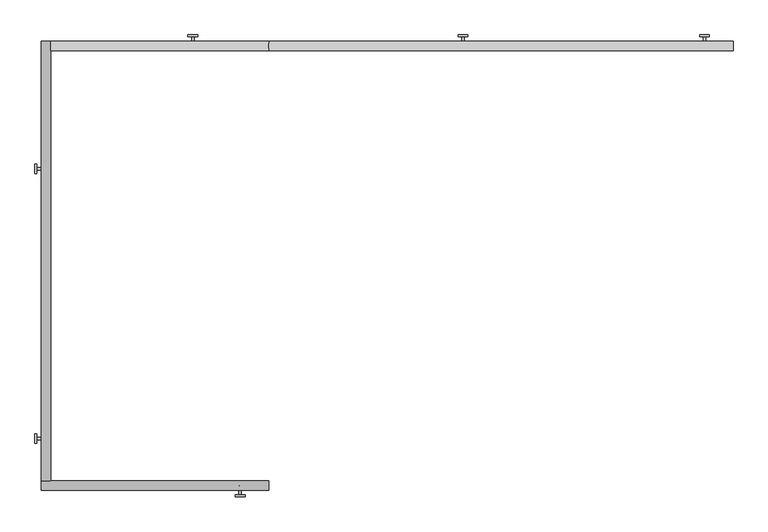
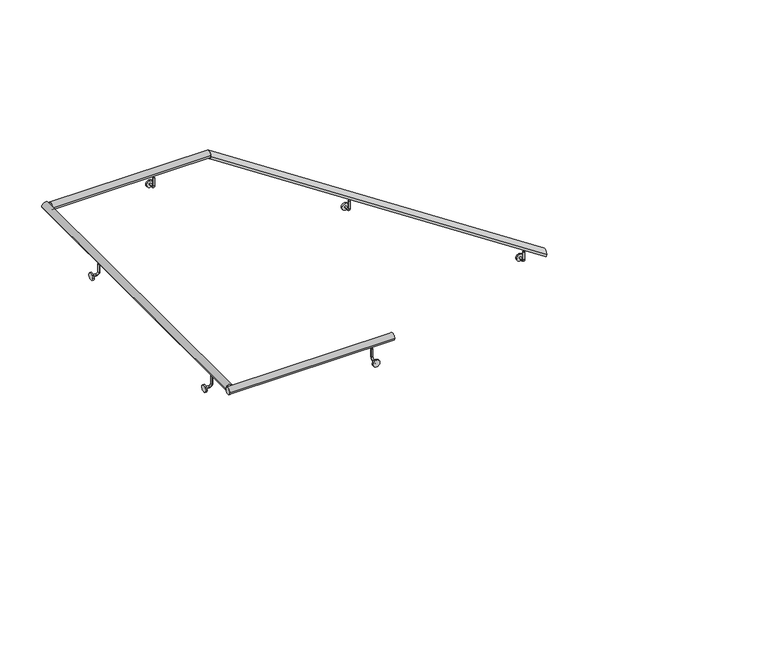
"""IFC4 building model written with IfcOpenShell, lengths in millimetres: railing geometry."""

from ifc_helpers import new_model, si_unit, point, frame, frame_2d, origin, place, context, project, spatial, circle_curve, ellipse_curve, trimmed, segment, composite_curve, outline, extrude, source, transform, mapped, element, save
from ifc_brep_helpers import plane_surface, cylinder_surface, revolved_surface, advanced_brep


def railing_2f2e9fd8(model_context):
    return source(origin(), model_context, "Body", "SolidModel", [
        advanced_brep(
        [(-47841.1127262, 17739.1574868, 1147.8451634), (-47841.1127262, 17789.1574868, 1147.8451634), (-50271.1127262, 17739.1574868, 2747.8451634), (-50271.1127262, 17789.1574868, 2747.8451634)],
        [
            (0, 1, ellipse_curve(frame((-47841.1127262, 17764.1574868, 1147.8451634), z_axis=(1.0, 0.0, 0.0), x_axis=(0.0, 0.0, -1.0)), 29.9326144, 25.0)),
            (1, 0, ellipse_curve(frame((-47841.1127262, 17764.1574868, 1147.8451634), z_axis=(1.0, 0.0, 0.0), x_axis=(0.0, 0.0, -1.0)), 29.9326144, 25.0)),
            (2, 3, ellipse_curve(frame((-50271.1127262, 17764.1574868, 2747.8451634), z_axis=(-1.0, 0.0, 0.0), x_axis=(0.0, 0.0, -1.0)), 29.9326144, 25.0)),
            (3, 2, ellipse_curve(frame((-50271.1127262, 17764.1574868, 2747.8451634), z_axis=(-1.0, 0.0, 0.0), x_axis=(0.0, 0.0, -1.0)), 29.9326144, 25.0)),
            (0, 2),
            (3, 1),
        ],
        [
            plane_surface(frame((-47841.1127262, 17764.1574868, 1177.7777778), z_axis=(1.0, 0.0, 0.0), x_axis=(0.0, -1.0, 0.0))),
            plane_surface(frame((-50271.1127262, 17764.1574868, 2777.7777778), z_axis=(-1.0, 0.0, 0.0), x_axis=(0.0, -1.0, 0.0))),
            cylinder_surface(frame((-47854.8610286, 17764.1574868, 1156.8975435), z_axis=(0.8352093694289686, 0.0, -0.5499320950972626), x_axis=(0.0, 1.0, 0.0)), 25.0),
        ],
        [
            (0, [[1, 2]]),
            (1, [[3, 4]]),
            (2, [[-1, 5, -4, 6]]),
            (2, [[-2, -6, -3, -5]]),
        ],
    ),
        advanced_brep(
        [(-50271.1127262, 17739.1574868, 2752.7777778), (-50271.1127262, 17789.1574868, 2752.7777778), (-51413.5127262, 17739.1574868, 2752.7777778), (-51413.5127262, 17789.1574868, 2752.7777778)],
        [
            (0, 1, circle_curve(frame((-50271.1127262, 17764.1574868, 2752.7777778), z_axis=(1.0, 0.0, 0.0), x_axis=(0.0, 1.0, 0.0)), 25.0)),
            (1, 0, circle_curve(frame((-50271.1127262, 17764.1574868, 2752.7777778), z_axis=(1.0, 0.0, 0.0), x_axis=(0.0, 1.0, 0.0)), 25.0)),
            (2, 3, circle_curve(frame((-51413.5127262, 17764.1574868, 2752.7777778), z_axis=(-1.0, 0.0, 0.0), x_axis=(0.0, 1.0, 0.0)), 25.0)),
            (3, 2, circle_curve(frame((-51413.5127262, 17764.1574868, 2752.7777778), z_axis=(-1.0, 0.0, 0.0), x_axis=(0.0, 1.0, 0.0)), 25.0)),
            (0, 2),
            (3, 1),
        ],
        [
            plane_surface(frame((-50271.1127262, 17764.1574868, 2777.7777778), z_axis=(1.0, 0.0, 0.0), x_axis=(0.0, -1.0, 0.0))),
            plane_surface(frame((-51413.5127262, 17764.1574868, 2777.7777778), z_axis=(-1.0, 0.0, 0.0), x_axis=(0.0, -1.0, 0.0))),
            cylinder_surface(frame((-50271.1127262, 17764.1574868, 2752.7777778), z_axis=(1.0, 0.0, 0.0), x_axis=(0.0, 1.0, 0.0)), 25.0),
        ],
        [
            (0, [[1, 2]]),
            (1, [[3, 4]]),
            (2, [[-1, 5, -4, 6]]),
            (2, [[-2, -6, -3, -5]]),
        ],
    ),
        advanced_brep(
        [(-51413.5127262, 17789.1574868, 2752.7777778), (-51463.5127262, 17789.1574868, 2752.7777778), (-51413.5127262, 15484.3587092, 2752.7777778), (-51463.5127262, 15484.3587092, 2752.7777778)],
        [
            (0, 1, circle_curve(frame((-51438.5127262, 17789.1574868, 2752.7777778), z_axis=(0.0, 1.0, 0.0), x_axis=(-1.0, 0.0, 0.0)), 25.0)),
            (1, 0, circle_curve(frame((-51438.5127262, 17789.1574868, 2752.7777778), z_axis=(0.0, 1.0, 0.0), x_axis=(-1.0, 0.0, 0.0)), 25.0)),
            (2, 3, circle_curve(frame((-51438.5127262, 15484.3587092, 2752.7777778), z_axis=(0.0, -1.0, 0.0), x_axis=(-1.0, 0.0, 0.0)), 25.0)),
            (3, 2, circle_curve(frame((-51438.5127262, 15484.3587092, 2752.7777778), z_axis=(0.0, -1.0, 0.0), x_axis=(-1.0, 0.0, 0.0)), 25.0)),
            (0, 2),
            (3, 1),
        ],
        [
            plane_surface(frame((-51438.5127262, 17789.1574868, 2777.7777778), z_axis=(0.0, 1.0, 0.0), x_axis=(0.0, 0.0, -1.0))),
            plane_surface(frame((-51438.5127262, 15484.3587092, 2777.7777778), z_axis=(0.0, -1.0, 0.0), x_axis=(0.0, 0.0, -1.0))),
            cylinder_surface(frame((-51438.5127262, 17789.1574868, 2752.7777778), z_axis=(0.0, 1.0, 0.0), x_axis=(-1.0, 0.0, 0.0)), 25.0),
        ],
        [
            (0, [[1, 2]]),
            (1, [[3, 4]]),
            (2, [[-1, 5, -4, 6]]),
            (2, [[-2, -6, -3, -5]]),
        ],
    ),
        advanced_brep(
        [(-51463.5127262, 15484.3587092, 2752.7777778), (-51463.5127262, 15434.3587092, 2752.7777778), (-50271.1127262, 15484.3587092, 2752.7777778), (-50271.1127262, 15434.3587092, 2752.7777778)],
        [
            (0, 1, circle_curve(frame((-51463.5127262, 15459.3587092, 2752.7777778), z_axis=(-1.0, 0.0, 0.0), x_axis=(0.0, -1.0, 0.0)), 25.0)),
            (1, 0, circle_curve(frame((-51463.5127262, 15459.3587092, 2752.7777778), z_axis=(-1.0, 0.0, 0.0), x_axis=(0.0, -1.0, 0.0)), 25.0)),
            (2, 3, circle_curve(frame((-50271.1127262, 15459.3587092, 2752.7777778), z_axis=(1.0, 0.0, 0.0), x_axis=(0.0, -1.0, 0.0)), 25.0)),
            (3, 2, circle_curve(frame((-50271.1127262, 15459.3587092, 2752.7777778), z_axis=(1.0, 0.0, 0.0), x_axis=(0.0, -1.0, 0.0)), 25.0)),
            (0, 2),
            (3, 1),
        ],
        [
            plane_surface(frame((-51463.5127262, 15459.3587092, 2777.7777778), z_axis=(-1.0, 0.0, 0.0), x_axis=(0.0, 1.0, 0.0))),
            plane_surface(frame((-50271.1127262, 15459.3587092, 2777.7777778), z_axis=(1.0, 0.0, 0.0), x_axis=(0.0, 1.0, 0.0))),
            cylinder_surface(frame((-51463.5127262, 15459.3587092, 2752.7777778), z_axis=(-1.0, 0.0, 0.0), x_axis=(0.0, -1.0, 0.0)), 25.0),
        ],
        [
            (0, [[1, 2]]),
            (1, [[3, 4]]),
            (2, [[-1, 5, -4, 6]]),
            (2, [[-2, -6, -3, -5]]),
        ],
    ),
        advanced_brep(
        [(-51438.5127262, 15712.2284647, 2708.7277778), (-51438.5127262, 15699.5284647, 2708.7277778), (-51438.5127262, 15712.2284647, 2651.5777778), (-51438.5127262, 15699.5284647, 2651.5777778), (-51457.5627262, 15699.5284647, 2632.5277778), (-51457.5627262, 15712.2284647, 2632.5277778), (-51486.1377262, 15712.2284647, 2632.5277778), (-51486.1377262, 15699.5284647, 2632.5277778)],
        [
            (0, 1, circle_curve(frame((-51438.5127262, 15705.8784647, 2708.7277778), z_axis=(0.0, 0.0, 1.0), x_axis=(0.0, -1.0, 0.0)), 6.35)),
            (1, 0, circle_curve(frame((-51438.5127262, 15705.8784647, 2708.7277778), z_axis=(0.0, 0.0, 1.0), x_axis=(0.0, -1.0, 0.0)), 6.35)),
            (0, 2),
            (2, 3, circle_curve(frame((-51438.5127262, 15705.8784647, 2651.5777778), z_axis=(0.0, 0.0, 1.0), x_axis=(0.0, -1.0, 0.0)), 6.35)),
            (3, 1),
            (3, 2, circle_curve(frame((-51438.5127262, 15705.8784647, 2651.5777778), z_axis=(0.0, 0.0, 1.0), x_axis=(0.0, -1.0, 0.0)), 6.35)),
            (4, 3, circle_curve(frame((-51457.5627262, 15699.5284647, 2651.5777778), z_axis=(0.0, -1.0, 0.0), x_axis=(1.0, 0.0, 0.0)), 19.05)),
            (2, 5, circle_curve(frame((-51457.5627262, 15712.2284647, 2651.5777778), z_axis=(0.0, 1.0, 0.0), x_axis=(1.0, 0.0, 0.0)), 19.05)),
            (5, 4, circle_curve(frame((-51457.5627262, 15705.8784647, 2632.5277778), z_axis=(1.0, 0.0, 0.0), x_axis=(0.0, -1.0, 0.0)), 6.35)),
            (4, 5, circle_curve(frame((-51457.5627262, 15705.8784647, 2632.5277778), z_axis=(1.0, 0.0, 0.0), x_axis=(0.0, -1.0, 0.0)), 6.35)),
            (6, 7, circle_curve(frame((-51486.1377262, 15705.8784647, 2632.5277778), z_axis=(-1.0, 0.0, 0.0), x_axis=(0.0, -1.0, 0.0)), 6.35)),
            (7, 6, circle_curve(frame((-51486.1377262, 15705.8784647, 2632.5277778), z_axis=(-1.0, 0.0, 0.0), x_axis=(0.0, -1.0, 0.0)), 6.35)),
            (5, 6),
            (7, 4),
        ],
        [
            plane_surface(frame((-51438.5127262, 15699.5284647, 2708.7277778), z_axis=(0.0, 0.0, 1.0), x_axis=(-1.0, 0.0, 0.0))),
            cylinder_surface(frame((-51438.5127262, 15705.8784647, 2708.7277778), z_axis=(0.0, 0.0, 1.0), x_axis=(0.0, -1.0, 0.0)), 6.35),
            revolved_surface(trimmed(ellipse_curve(frame((-51438.5127262, 15705.8784647, 2651.5777778), z_axis=(0.0, 0.0, 1.0), x_axis=(0.0, -1.0, 0.0)), 6.35, 6.35), [point((-51438.5127262, 15712.2284647, 2651.5777778))], [point((-51438.5127262, 15699.5284647, 2651.5777778))], True, "CARTESIAN"), (-51457.5627262, 15705.8784647, 2651.5777778), (0.0, 1.0, 0.0)),
            revolved_surface(trimmed(ellipse_curve(frame((-51438.5127262, 15705.8784647, 2651.5777778), z_axis=(0.0, 0.0, 1.0), x_axis=(0.0, -1.0, 0.0)), 6.35, 6.35), [point((-51438.5127262, 15699.5284647, 2651.5777778))], [point((-51438.5127262, 15712.2284647, 2651.5777778))], True, "CARTESIAN"), (-51457.5627262, 15705.8784647, 2651.5777778), (0.0, 1.0, 0.0)),
            plane_surface(frame((-51486.1377262, 15705.8784647, 2626.1777778), z_axis=(-1.0, 0.0, 0.0), x_axis=(0.0, -1.0, 0.0))),
            cylinder_surface(frame((-51457.5627262, 15705.8784647, 2632.5277778), z_axis=(1.0, 0.0, 0.0), x_axis=(0.0, -1.0, 0.0)), 6.35),
        ],
        [
            (0, [[1, 2]]),
            (1, [[-1, 3, 4, 5]]),
            (1, [[-2, -5, 6, -3]]),
            (2, [[7, -4, 8, 9]]),
            (3, [[-8, -6, -7, 10]]),
            (4, [[11, 12]]),
            (5, [[-9, 13, -12, 14]]),
            (5, [[-10, -14, -11, -13]]),
        ],
    ),
        extrude(outline(composite_curve([segment(trimmed(circle_curve(frame_2d((15705.8784647, 2632.5277778)), 25.4), [point((15680.4784647, 2632.5277778))], [point((15731.2784647, 2632.5277778))], False, "CARTESIAN"), True, "CONTINUOUS"), segment(trimmed(circle_curve(frame_2d((15705.8784647, 2632.5277778)), 25.4), [point((15731.2784647, 2632.5277778))], [point((15680.4784647, 2632.5277778))], False, "CARTESIAN"), True, "CONTINUOUS")], self_intersect=False)), frame((-51495.6627262, 0.0, 0.0), z_axis=(1.0, 0.0, 0.0), x_axis=(0.0, 1.0, 0.0)), (0.0, 0.0, 1.0), 9.525),
        advanced_brep(
        [(-51438.5127262, 17126.1482202, 2708.7277778), (-51438.5127262, 17113.4482202, 2708.7277778), (-51438.5127262, 17126.1482202, 2651.5777778), (-51438.5127262, 17113.4482202, 2651.5777778), (-51457.5627262, 17113.4482202, 2632.5277778), (-51457.5627262, 17126.1482202, 2632.5277778), (-51486.1377262, 17126.1482202, 2632.5277778), (-51486.1377262, 17113.4482202, 2632.5277778)],
        [
            (0, 1, circle_curve(frame((-51438.5127262, 17119.7982202, 2708.7277778), z_axis=(0.0, 0.0, 1.0), x_axis=(0.0, -1.0, 0.0)), 6.35)),
            (1, 0, circle_curve(frame((-51438.5127262, 17119.7982202, 2708.7277778), z_axis=(0.0, 0.0, 1.0), x_axis=(0.0, -1.0, 0.0)), 6.35)),
            (0, 2),
            (2, 3, circle_curve(frame((-51438.5127262, 17119.7982202, 2651.5777778), z_axis=(0.0, 0.0, 1.0), x_axis=(0.0, -1.0, 0.0)), 6.35)),
            (3, 1),
            (3, 2, circle_curve(frame((-51438.5127262, 17119.7982202, 2651.5777778), z_axis=(0.0, 0.0, 1.0), x_axis=(0.0, -1.0, 0.0)), 6.35)),
            (4, 3, circle_curve(frame((-51457.5627262, 17113.4482202, 2651.5777778), z_axis=(0.0, -1.0, 0.0), x_axis=(1.0, 0.0, 0.0)), 19.05)),
            (2, 5, circle_curve(frame((-51457.5627262, 17126.1482202, 2651.5777778), z_axis=(0.0, 1.0, 0.0), x_axis=(1.0, 0.0, 0.0)), 19.05)),
            (5, 4, circle_curve(frame((-51457.5627262, 17119.7982202, 2632.5277778), z_axis=(1.0, 0.0, 0.0), x_axis=(0.0, -1.0, 0.0)), 6.35)),
            (4, 5, circle_curve(frame((-51457.5627262, 17119.7982202, 2632.5277778), z_axis=(1.0, 0.0, 0.0), x_axis=(0.0, -1.0, 0.0)), 6.35)),
            (6, 7, circle_curve(frame((-51486.1377262, 17119.7982202, 2632.5277778), z_axis=(-1.0, 0.0, 0.0), x_axis=(0.0, -1.0, 0.0)), 6.35)),
            (7, 6, circle_curve(frame((-51486.1377262, 17119.7982202, 2632.5277778), z_axis=(-1.0, 0.0, 0.0), x_axis=(0.0, -1.0, 0.0)), 6.35)),
            (5, 6),
            (7, 4),
        ],
        [
            plane_surface(frame((-51438.5127262, 17113.4482202, 2708.7277778), z_axis=(0.0, 0.0, 1.0), x_axis=(-1.0, 0.0, 0.0))),
            cylinder_surface(frame((-51438.5127262, 17119.7982202, 2708.7277778), z_axis=(0.0, 0.0, 1.0), x_axis=(0.0, -1.0, 0.0)), 6.35),
            revolved_surface(trimmed(ellipse_curve(frame((-51438.5127262, 17119.7982202, 2651.5777778), z_axis=(0.0, 0.0, 1.0), x_axis=(0.0, -1.0, 0.0)), 6.35, 6.35), [point((-51438.5127262, 17126.1482202, 2651.5777778))], [point((-51438.5127262, 17113.4482202, 2651.5777778))], True, "CARTESIAN"), (-51457.5627262, 17119.7982202, 2651.5777778), (0.0, 1.0, 0.0)),
            revolved_surface(trimmed(ellipse_curve(frame((-51438.5127262, 17119.7982202, 2651.5777778), z_axis=(0.0, 0.0, 1.0), x_axis=(0.0, -1.0, 0.0)), 6.35, 6.35), [point((-51438.5127262, 17113.4482202, 2651.5777778))], [point((-51438.5127262, 17126.1482202, 2651.5777778))], True, "CARTESIAN"), (-51457.5627262, 17119.7982202, 2651.5777778), (0.0, 1.0, 0.0)),
            plane_surface(frame((-51486.1377262, 17119.7982202, 2626.1777778), z_axis=(-1.0, 0.0, 0.0), x_axis=(0.0, -1.0, 0.0))),
            cylinder_surface(frame((-51457.5627262, 17119.7982202, 2632.5277778), z_axis=(1.0, 0.0, 0.0), x_axis=(0.0, -1.0, 0.0)), 6.35),
        ],
        [
            (0, [[1, 2]]),
            (1, [[-1, 3, 4, 5]]),
            (1, [[-2, -5, 6, -3]]),
            (2, [[7, -4, 8, 9]]),
            (3, [[-8, -6, -7, 10]]),
            (4, [[11, 12]]),
            (5, [[-9, 13, -12, 14]]),
            (5, [[-10, -14, -11, -13]]),
        ],
    ),
        extrude(outline(composite_curve([segment(trimmed(circle_curve(frame_2d((17119.7982202, 2632.5277778)), 25.4), [point((17094.3982202, 2632.5277778))], [point((17145.1982202, 2632.5277778))], False, "CARTESIAN"), True, "CONTINUOUS"), segment(trimmed(circle_curve(frame_2d((17119.7982202, 2632.5277778)), 25.4), [point((17145.1982202, 2632.5277778))], [point((17094.3982202, 2632.5277778))], False, "CARTESIAN"), True, "CONTINUOUS")], self_intersect=False)), frame((-51495.6627262, 0.0, 0.0), z_axis=(1.0, 0.0, 0.0), x_axis=(0.0, 1.0, 0.0)), (0.0, 0.0, 1.0), 9.525),
        advanced_brep(
        [(-50662.6022373, 17764.1574868, 2708.7277778), (-50675.3022373, 17764.1574868, 2708.7277778), (-50662.6022373, 17764.1574868, 2651.5777778), (-50675.3022373, 17764.1574868, 2651.5777778), (-50675.3022373, 17783.2074868, 2632.5277778), (-50662.6022373, 17783.2074868, 2632.5277778), (-50662.6022373, 17811.7824868, 2632.5277778), (-50675.3022373, 17811.7824868, 2632.5277778)],
        [
            (0, 1, circle_curve(frame((-50668.9522373, 17764.1574868, 2708.7277778), z_axis=(0.0, 0.0, 1.0), x_axis=(-1.0, 0.0, 0.0)), 6.35)),
            (1, 0, circle_curve(frame((-50668.9522373, 17764.1574868, 2708.7277778), z_axis=(0.0, 0.0, 1.0), x_axis=(-1.0, 0.0, 0.0)), 6.35)),
            (0, 2),
            (2, 3, circle_curve(frame((-50668.9522373, 17764.1574868, 2651.5777778), z_axis=(0.0, 0.0, 1.0), x_axis=(-1.0, 0.0, 0.0)), 6.35)),
            (3, 1),
            (3, 2, circle_curve(frame((-50668.9522373, 17764.1574868, 2651.5777778), z_axis=(0.0, 0.0, 1.0), x_axis=(-1.0, 0.0, 0.0)), 6.35)),
            (4, 3, circle_curve(frame((-50675.3022373, 17783.2074868, 2651.5777778), z_axis=(-1.0, 0.0, 0.0), x_axis=(0.0, -1.0, 0.0)), 19.05)),
            (2, 5, circle_curve(frame((-50662.6022373, 17783.2074868, 2651.5777778), z_axis=(1.0, 0.0, 0.0), x_axis=(0.0, -1.0, 0.0)), 19.05)),
            (5, 4, circle_curve(frame((-50668.9522373, 17783.2074868, 2632.5277778), z_axis=(0.0, -1.0, 0.0), x_axis=(-1.0, 0.0, 0.0)), 6.35)),
            (4, 5, circle_curve(frame((-50668.9522373, 17783.2074868, 2632.5277778), z_axis=(0.0, -1.0, 0.0), x_axis=(-1.0, 0.0, 0.0)), 6.35)),
            (6, 7, circle_curve(frame((-50668.9522373, 17811.7824868, 2632.5277778), z_axis=(0.0, 1.0, 0.0), x_axis=(-1.0, 0.0, 0.0)), 6.35)),
            (7, 6, circle_curve(frame((-50668.9522373, 17811.7824868, 2632.5277778), z_axis=(0.0, 1.0, 0.0), x_axis=(-1.0, 0.0, 0.0)), 6.35)),
            (5, 6),
            (7, 4),
        ],
        [
            plane_surface(frame((-50675.3022373, 17764.1574868, 2708.7277778), z_axis=(0.0, 0.0, 1.0), x_axis=(0.0, 1.0, 0.0))),
            cylinder_surface(frame((-50668.9522373, 17764.1574868, 2708.7277778), z_axis=(0.0, 0.0, 1.0), x_axis=(-1.0, 0.0, 0.0)), 6.35),
            revolved_surface(trimmed(ellipse_curve(frame((-50668.9522373, 17764.1574868, 2651.5777778), z_axis=(0.0, 0.0, 1.0), x_axis=(-1.0, 0.0, 0.0)), 6.35, 6.35), [point((-50662.6022373, 17764.1574868, 2651.5777778))], [point((-50675.3022373, 17764.1574868, 2651.5777778))], True, "CARTESIAN"), (-50668.9522373, 17783.2074868, 2651.5777778), (1.0, 0.0, 0.0)),
            revolved_surface(trimmed(ellipse_curve(frame((-50668.9522373, 17764.1574868, 2651.5777778), z_axis=(0.0, 0.0, 1.0), x_axis=(-1.0, 0.0, 0.0)), 6.35, 6.35), [point((-50675.3022373, 17764.1574868, 2651.5777778))], [point((-50662.6022373, 17764.1574868, 2651.5777778))], True, "CARTESIAN"), (-50668.9522373, 17783.2074868, 2651.5777778), (1.0, 0.0, 0.0)),
            plane_surface(frame((-50668.9522373, 17811.7824868, 2626.1777778), z_axis=(0.0, 1.0, 0.0), x_axis=(-1.0, 0.0, 0.0))),
            cylinder_surface(frame((-50668.9522373, 17783.2074868, 2632.5277778), z_axis=(0.0, -1.0, 0.0), x_axis=(-1.0, 0.0, 0.0)), 6.35),
        ],
        [
            (0, [[1, 2]]),
            (1, [[-1, 3, 4, 5]]),
            (1, [[-2, -5, 6, -3]]),
            (2, [[7, -4, 8, 9]]),
            (3, [[-8, -6, -7, 10]]),
            (4, [[11, 12]]),
            (5, [[-9, 13, -12, 14]]),
            (5, [[-10, -14, -11, -13]]),
        ],
    ),
        extrude(outline(composite_curve([segment(trimmed(circle_curve(frame_2d((2632.5277778, -50668.9522373)), 25.4), [point((2632.5277778, -50694.3522373))], [point((2632.5277778, -50643.5522373))], False, "CARTESIAN"), True, "CONTINUOUS"), segment(trimmed(circle_curve(frame_2d((2632.5277778, -50668.9522373)), 25.4), [point((2632.5277778, -50643.5522373))], [point((2632.5277778, -50694.3522373))], False, "CARTESIAN"), True, "CONTINUOUS")], self_intersect=False)), frame((0.0, 17811.7824868, 0.0), z_axis=(0.0, 1.0, 0.0), x_axis=(0.0, 0.0, 1.0)), (0.0, 0.0, 1.0), 9.525),
        advanced_brep(
        [(-49248.6824817, 17764.1574868, 2039.7037485), (-49261.3824817, 17764.1574868, 2039.7037485), (-49248.6824817, 17764.1574868, 1982.5537485), (-49261.3824817, 17764.1574868, 1982.5537485), (-49261.3824817, 17783.2074868, 1963.5037485), (-49248.6824817, 17783.2074868, 1963.5037485), (-49248.6824817, 17811.7824868, 1963.5037485), (-49261.3824817, 17811.7824868, 1963.5037485)],
        [
            (0, 1, circle_curve(frame((-49255.0324817, 17764.1574868, 2039.7037485), z_axis=(0.0, 0.0, 1.0), x_axis=(-1.0, 0.0, 0.0)), 6.35)),
            (1, 0, circle_curve(frame((-49255.0324817, 17764.1574868, 2039.7037485), z_axis=(0.0, 0.0, 1.0), x_axis=(-1.0, 0.0, 0.0)), 6.35)),
            (0, 2),
            (2, 3, circle_curve(frame((-49255.0324817, 17764.1574868, 1982.5537485), z_axis=(0.0, 0.0, 1.0), x_axis=(-1.0, 0.0, 0.0)), 6.35)),
            (3, 1),
            (3, 2, circle_curve(frame((-49255.0324817, 17764.1574868, 1982.5537485), z_axis=(0.0, 0.0, 1.0), x_axis=(-1.0, 0.0, 0.0)), 6.35)),
            (4, 3, circle_curve(frame((-49261.3824817, 17783.2074868, 1982.5537485), z_axis=(-1.0, 0.0, 0.0), x_axis=(0.0, -1.0, 0.0)), 19.05)),
            (2, 5, circle_curve(frame((-49248.6824817, 17783.2074868, 1982.5537485), z_axis=(1.0, 0.0, 0.0), x_axis=(0.0, -1.0, 0.0)), 19.05)),
            (5, 4, circle_curve(frame((-49255.0324817, 17783.2074868, 1963.5037485), z_axis=(0.0, -1.0, 0.0), x_axis=(-1.0, 0.0, 0.0)), 6.35)),
            (4, 5, circle_curve(frame((-49255.0324817, 17783.2074868, 1963.5037485), z_axis=(0.0, -1.0, 0.0), x_axis=(-1.0, 0.0, 0.0)), 6.35)),
            (6, 7, circle_curve(frame((-49255.0324817, 17811.7824868, 1963.5037485), z_axis=(0.0, 1.0, 0.0), x_axis=(-1.0, 0.0, 0.0)), 6.35)),
            (7, 6, circle_curve(frame((-49255.0324817, 17811.7824868, 1963.5037485), z_axis=(0.0, 1.0, 0.0), x_axis=(-1.0, 0.0, 0.0)), 6.35)),
            (5, 6),
            (7, 4),
        ],
        [
            plane_surface(frame((-49261.3824817, 17764.1574868, 2039.7037485), z_axis=(0.0, 0.0, 1.0), x_axis=(0.0, 1.0, 0.0))),
            cylinder_surface(frame((-49255.0324817, 17764.1574868, 2039.7037485), z_axis=(0.0, 0.0, 1.0), x_axis=(-1.0, 0.0, 0.0)), 6.35),
            revolved_surface(trimmed(ellipse_curve(frame((-49255.0324817, 17764.1574868, 1982.5537485), z_axis=(0.0, 0.0, 1.0), x_axis=(-1.0, 0.0, 0.0)), 6.35, 6.35), [point((-49248.6824817, 17764.1574868, 1982.5537485))], [point((-49261.3824817, 17764.1574868, 1982.5537485))], True, "CARTESIAN"), (-49255.0324817, 17783.2074868, 1982.5537485), (1.0, 0.0, 0.0)),
            revolved_surface(trimmed(ellipse_curve(frame((-49255.0324817, 17764.1574868, 1982.5537485), z_axis=(0.0, 0.0, 1.0), x_axis=(-1.0, 0.0, 0.0)), 6.35, 6.35), [point((-49261.3824817, 17764.1574868, 1982.5537485))], [point((-49248.6824817, 17764.1574868, 1982.5537485))], True, "CARTESIAN"), (-49255.0324817, 17783.2074868, 1982.5537485), (1.0, 0.0, 0.0)),
            plane_surface(frame((-49255.0324817, 17811.7824868, 1957.1537485), z_axis=(0.0, 1.0, 0.0), x_axis=(-1.0, 0.0, 0.0))),
            cylinder_surface(frame((-49255.0324817, 17783.2074868, 1963.5037485), z_axis=(0.0, -1.0, 0.0), x_axis=(-1.0, 0.0, 0.0)), 6.35),
        ],
        [
            (0, [[1, 2]]),
            (1, [[-1, 3, 4, 5]]),
            (1, [[-2, -5, 6, -3]]),
            (2, [[7, -4, 8, 9]]),
            (3, [[-8, -6, -7, 10]]),
            (4, [[11, 12]]),
            (5, [[-9, 13, -12, 14]]),
            (5, [[-10, -14, -11, -13]]),
        ],
    ),
        extrude(outline(composite_curve([segment(trimmed(circle_curve(frame_2d((1963.5037485, -49255.0324817)), 25.4), [point((1963.5037485, -49280.4324817))], [point((1963.5037485, -49229.6324817))], False, "CARTESIAN"), True, "CONTINUOUS"), segment(trimmed(circle_curve(frame_2d((1963.5037485, -49255.0324817)), 25.4), [point((1963.5037485, -49229.6324817))], [point((1963.5037485, -49280.4324817))], False, "CARTESIAN"), True, "CONTINUOUS")], self_intersect=False)), frame((0.0, 17811.7824868, 0.0), z_axis=(0.0, 1.0, 0.0), x_axis=(0.0, 0.0, 1.0)), (0.0, 0.0, 1.0), 9.525),
        advanced_brep(
        [(-50427.4627262, 15459.3587092, 2708.7277778), (-50414.7627262, 15459.3587092, 2708.7277778), (-50427.4627262, 15459.3587092, 2651.5777778), (-50414.7627262, 15459.3587092, 2651.5777778), (-50414.7627262, 15440.3087092, 2632.5277778), (-50427.4627262, 15440.3087092, 2632.5277778), (-50427.4627262, 15411.7337092, 2632.5277778), (-50414.7627262, 15411.7337092, 2632.5277778)],
        [
            (0, 1, circle_curve(frame((-50421.1127262, 15459.3587092, 2708.7277778), z_axis=(0.0, 0.0, 1.0), x_axis=(1.0, 0.0, 0.0)), 6.35)),
            (1, 0, circle_curve(frame((-50421.1127262, 15459.3587092, 2708.7277778), z_axis=(0.0, 0.0, 1.0), x_axis=(1.0, 0.0, 0.0)), 6.35)),
            (0, 2),
            (2, 3, circle_curve(frame((-50421.1127262, 15459.3587092, 2651.5777778), z_axis=(0.0, 0.0, 1.0), x_axis=(1.0, 0.0, 0.0)), 6.35)),
            (3, 1),
            (3, 2, circle_curve(frame((-50421.1127262, 15459.3587092, 2651.5777778), z_axis=(0.0, 0.0, 1.0), x_axis=(1.0, 0.0, 0.0)), 6.35)),
            (4, 3, circle_curve(frame((-50414.7627262, 15440.3087092, 2651.5777778), z_axis=(1.0, 0.0, 0.0), x_axis=(0.0, 1.0, 0.0)), 19.05)),
            (2, 5, circle_curve(frame((-50427.4627262, 15440.3087092, 2651.5777778), z_axis=(-1.0, 0.0, 0.0), x_axis=(0.0, 1.0, 0.0)), 19.05)),
            (5, 4, circle_curve(frame((-50421.1127262, 15440.3087092, 2632.5277778), z_axis=(0.0, 1.0, 0.0), x_axis=(1.0, 0.0, 0.0)), 6.35)),
            (4, 5, circle_curve(frame((-50421.1127262, 15440.3087092, 2632.5277778), z_axis=(0.0, 1.0, 0.0), x_axis=(1.0, 0.0, 0.0)), 6.35)),
            (6, 7, circle_curve(frame((-50421.1127262, 15411.7337092, 2632.5277778), z_axis=(0.0, -1.0, 0.0), x_axis=(1.0, 0.0, 0.0)), 6.35)),
            (7, 6, circle_curve(frame((-50421.1127262, 15411.7337092, 2632.5277778), z_axis=(0.0, -1.0, 0.0), x_axis=(1.0, 0.0, 0.0)), 6.35)),
            (5, 6),
            (7, 4),
        ],
        [
            plane_surface(frame((-50414.7627262, 15459.3587092, 2708.7277778), z_axis=(0.0, 0.0, 1.0), x_axis=(0.0, -1.0, 0.0))),
            cylinder_surface(frame((-50421.1127262, 15459.3587092, 2708.7277778), z_axis=(0.0, 0.0, 1.0), x_axis=(1.0, 0.0, 0.0)), 6.35),
            revolved_surface(trimmed(ellipse_curve(frame((-50421.1127262, 15459.3587092, 2651.5777778), z_axis=(0.0, 0.0, 1.0), x_axis=(1.0, 0.0, 0.0)), 6.35, 6.35), [point((-50427.4627262, 15459.3587092, 2651.5777778))], [point((-50414.7627262, 15459.3587092, 2651.5777778))], True, "CARTESIAN"), (-50421.1127262, 15440.3087092, 2651.5777778), (-1.0, 0.0, 0.0)),
            revolved_surface(trimmed(ellipse_curve(frame((-50421.1127262, 15459.3587092, 2651.5777778), z_axis=(0.0, 0.0, 1.0), x_axis=(1.0, 0.0, 0.0)), 6.35, 6.35), [point((-50414.7627262, 15459.3587092, 2651.5777778))], [point((-50427.4627262, 15459.3587092, 2651.5777778))], True, "CARTESIAN"), (-50421.1127262, 15440.3087092, 2651.5777778), (-1.0, 0.0, 0.0)),
            plane_surface(frame((-50421.1127262, 15411.7337092, 2626.1777778), z_axis=(0.0, -1.0, 0.0), x_axis=(1.0, 0.0, 0.0))),
            cylinder_surface(frame((-50421.1127262, 15440.3087092, 2632.5277778), z_axis=(0.0, 1.0, 0.0), x_axis=(1.0, 0.0, 0.0)), 6.35),
        ],
        [
            (0, [[1, 2]]),
            (1, [[-1, 3, 4, 5]]),
            (1, [[-2, -5, 6, -3]]),
            (2, [[7, -4, 8, 9]]),
            (3, [[-8, -6, -7, 10]]),
            (4, [[11, 12]]),
            (5, [[-9, 13, -12, 14]]),
            (5, [[-10, -14, -11, -13]]),
        ],
    ),
        extrude(outline(composite_curve([segment(trimmed(circle_curve(frame_2d((2632.5277778, -50421.1127262)), 25.4), [point((2632.5277778, -50395.7127262))], [point((2632.5277778, -50446.5127262))], False, "CARTESIAN"), True, "CONTINUOUS"), segment(trimmed(circle_curve(frame_2d((2632.5277778, -50421.1127262)), 25.4), [point((2632.5277778, -50446.5127262))], [point((2632.5277778, -50395.7127262))], False, "CARTESIAN"), True, "CONTINUOUS")], self_intersect=False)), frame((0.0, 15402.2087092, 0.0), z_axis=(0.0, 1.0, 0.0), x_axis=(0.0, 0.0, 1.0)), (0.0, 0.0, 1.0), 9.525),
        advanced_brep(
        [(-47984.7627262, 17764.1574868, 1207.4932099), (-47997.4627262, 17764.1574868, 1207.4932099), (-47984.7627262, 17764.1574868, 1150.3432099), (-47997.4627262, 17764.1574868, 1150.3432099), (-47997.4627262, 17783.2074868, 1131.2932099), (-47984.7627262, 17783.2074868, 1131.2932099), (-47984.7627262, 17811.7824868, 1131.2932099), (-47997.4627262, 17811.7824868, 1131.2932099)],
        [
            (0, 1, circle_curve(frame((-47991.1127262, 17764.1574868, 1207.4932099), z_axis=(0.0, 0.0, 1.0), x_axis=(-1.0, 0.0, 0.0)), 6.35)),
            (1, 0, circle_curve(frame((-47991.1127262, 17764.1574868, 1207.4932099), z_axis=(0.0, 0.0, 1.0), x_axis=(-1.0, 0.0, 0.0)), 6.35)),
            (0, 2),
            (2, 3, circle_curve(frame((-47991.1127262, 17764.1574868, 1150.3432099), z_axis=(0.0, 0.0, 1.0), x_axis=(-1.0, 0.0, 0.0)), 6.35)),
            (3, 1),
            (3, 2, circle_curve(frame((-47991.1127262, 17764.1574868, 1150.3432099), z_axis=(0.0, 0.0, 1.0), x_axis=(-1.0, 0.0, 0.0)), 6.35)),
            (4, 3, circle_curve(frame((-47997.4627262, 17783.2074868, 1150.3432099), z_axis=(-1.0, 0.0, 0.0), x_axis=(0.0, -1.0, 0.0)), 19.05)),
            (2, 5, circle_curve(frame((-47984.7627262, 17783.2074868, 1150.3432099), z_axis=(1.0, 0.0, 0.0), x_axis=(0.0, -1.0, 0.0)), 19.05)),
            (5, 4, circle_curve(frame((-47991.1127262, 17783.2074868, 1131.2932099), z_axis=(0.0, -1.0, 0.0), x_axis=(-1.0, 0.0, 0.0)), 6.35)),
            (4, 5, circle_curve(frame((-47991.1127262, 17783.2074868, 1131.2932099), z_axis=(0.0, -1.0, 0.0), x_axis=(-1.0, 0.0, 0.0)), 6.35)),
            (6, 7, circle_curve(frame((-47991.1127262, 17811.7824868, 1131.2932099), z_axis=(0.0, 1.0, 0.0), x_axis=(-1.0, 0.0, 0.0)), 6.35)),
            (7, 6, circle_curve(frame((-47991.1127262, 17811.7824868, 1131.2932099), z_axis=(0.0, 1.0, 0.0), x_axis=(-1.0, 0.0, 0.0)), 6.35)),
            (5, 6),
            (7, 4),
        ],
        [
            plane_surface(frame((-47997.4627262, 17764.1574868, 1207.4932099), z_axis=(0.0, 0.0, 1.0), x_axis=(0.0, 1.0, 0.0))),
            cylinder_surface(frame((-47991.1127262, 17764.1574868, 1207.4932099), z_axis=(0.0, 0.0, 1.0), x_axis=(-1.0, 0.0, 0.0)), 6.35),
            revolved_surface(trimmed(ellipse_curve(frame((-47991.1127262, 17764.1574868, 1150.3432099), z_axis=(0.0, 0.0, 1.0), x_axis=(-1.0, 0.0, 0.0)), 6.35, 6.35), [point((-47984.7627262, 17764.1574868, 1150.3432099))], [point((-47997.4627262, 17764.1574868, 1150.3432099))], True, "CARTESIAN"), (-47991.1127262, 17783.2074868, 1150.3432099), (1.0, 0.0, 0.0)),
            revolved_surface(trimmed(ellipse_curve(frame((-47991.1127262, 17764.1574868, 1150.3432099), z_axis=(0.0, 0.0, 1.0), x_axis=(-1.0, 0.0, 0.0)), 6.35, 6.35), [point((-47997.4627262, 17764.1574868, 1150.3432099))], [point((-47984.7627262, 17764.1574868, 1150.3432099))], True, "CARTESIAN"), (-47991.1127262, 17783.2074868, 1150.3432099), (1.0, 0.0, 0.0)),
            plane_surface(frame((-47991.1127262, 17811.7824868, 1124.9432099), z_axis=(0.0, 1.0, 0.0), x_axis=(-1.0, 0.0, 0.0))),
            cylinder_surface(frame((-47991.1127262, 17783.2074868, 1131.2932099), z_axis=(0.0, -1.0, 0.0), x_axis=(-1.0, 0.0, 0.0)), 6.35),
        ],
        [
            (0, [[1, 2]]),
            (1, [[-1, 3, 4, 5]]),
            (1, [[-2, -5, 6, -3]]),
            (2, [[7, -4, 8, 9]]),
            (3, [[-8, -6, -7, 10]]),
            (4, [[11, 12]]),
            (5, [[-9, 13, -12, 14]]),
            (5, [[-10, -14, -11, -13]]),
        ],
    ),
        extrude(outline(composite_curve([segment(trimmed(circle_curve(frame_2d((1131.2932099, -47991.1127262)), 25.4), [point((1131.2932099, -48016.5127262))], [point((1131.2932099, -47965.7127262))], False, "CARTESIAN"), True, "CONTINUOUS"), segment(trimmed(circle_curve(frame_2d((1131.2932099, -47991.1127262)), 25.4), [point((1131.2932099, -47965.7127262))], [point((1131.2932099, -48016.5127262))], False, "CARTESIAN"), True, "CONTINUOUS")], self_intersect=False)), frame((0.0, 17811.7824868, 0.0), z_axis=(0.0, 1.0, 0.0), x_axis=(0.0, 0.0, 1.0)), (0.0, 0.0, 1.0), 9.525),
    ])


if __name__ == "__main__":
    model = new_model("IFC4")
    model_context = context("Model", 3, world=origin())
    ifc_project = project(units=[si_unit("LENGTHUNIT", "METRE", prefix="MILLI")], contexts=[model_context])
    site = spatial("IfcSite", under=ifc_project)
    building = spatial("IfcBuilding", under=site)
    placement = place(None, origin())
    railing_shape = railing_2f2e9fd8(model_context)
    element("IfcRailing", 1, at=placement, inside=building, context=model_context, shape_type="MappedRepresentation", body=[
        mapped(railing_shape, transform((0.0, 0.0, 0.0), x_axis=(1.0, 0.0, 0.0), y_axis=(0.0, 1.0, 0.0), z_axis=(0.0, 0.0, 1.0))),
    ])
    save(model, "model.ifc")
